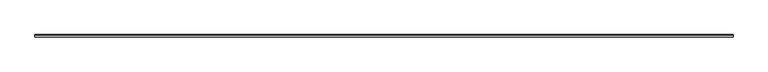
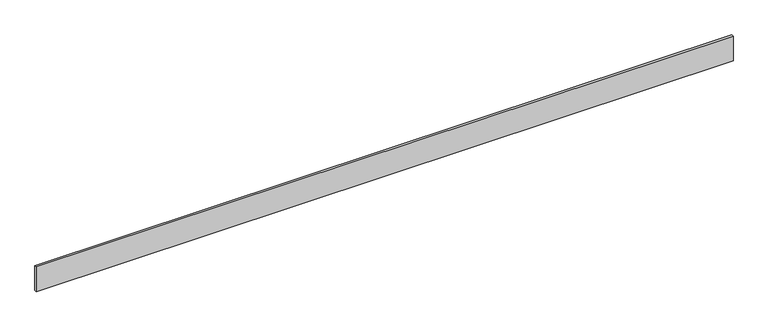
"""IFC4 building model written with IfcOpenShell, lengths in millimetres: proxy geometry, Generic Models 7:Generic Models 1:8:Generic Models 1:8 : Generic Models 7:Generic Models 1:337419:5 : Generic Models 7:Generic Models 1:8:Generic Models 1:8 : Generic Models 7:Generic Models 1:337419:315935."""

from ifc_helpers import new_model, si_unit, frame, origin, place, context, project, spatial, polyline, outline, extrude, source, transform, mapped, element, save


def generic_models_05c8018c(model_context):
    return source(origin(), model_context, "Body", "SweptSolid", [
        extrude(outline(polyline([(-579080.8776331, 3903.4402499), (-579080.0663873, 3902.6290041), (-579080.0663873, 3720.3062499), (-579095.9413873, 3720.3062499), (-579095.9413873, 3903.4402499), (-579080.8776331, 3903.4402499)])), frame((591306.0367239, 0.0, 0.0), z_axis=(1.0, 0.0, 0.0), x_axis=(0.0, 1.0, 0.0)), (0.0, 0.0, 1.0), 4876.8),
    ])


if __name__ == "__main__":
    model = new_model("IFC4")
    model_context = context("Model", 3, world=origin())
    ifc_project = project(units=[si_unit("LENGTHUNIT", "METRE", prefix="MILLI")], contexts=[model_context])
    site = spatial("IfcSite", under=ifc_project)
    building = spatial("IfcBuilding", under=site)
    placement = place(None, origin())
    generic_models_shape = generic_models_05c8018c(model_context)
    element("IfcBuildingElementProxy", 1, Name="Generic Models 7:Generic Models 1:8:Generic Models 1:8 : Generic Models 7:Generic Models 1:337419:5 : Generic Models 7:Generic Models 1:8:Generic Models 1:8 : Generic Models 7:Generic Models 1:337419:315935", ObjectType="Generic Models 7:Generic Models 1:8:Generic Models 1:8 : Generic Models 7:Generic Models 1:337419:5 : Generic Models 7:Generic Models 1:8:Generic Models 1:8 : Generic Models 7:Generic Models 1:337419:315935", at=placement, inside=building, context=model_context, shape_type="MappedRepresentation", body=[
        mapped(generic_models_shape, transform((0.0, 0.0, 0.0), x_axis=(1.0, 0.0, 0.0), y_axis=(0.0, 1.0, 0.0), z_axis=(0.0, 0.0, 1.0))),
    ])
    save(model, "model.ifc")

# Revit data of these elements
# Type "Generic Models 7:Generic Models 1:8:Generic Models 1:8 : Generic Models 7:Generic Models 1:337419:5 : Generic Models 7:Generic Models 1:8:Generic Models 1:8 : Generic Models 7:Generic Models 1:337419:315935"
#   NameOverride = "Generic Models 7:Generic Models 1:8:Generic Models 1:8 : Generic Models 7:Generic Models 1:337419:315935"
#   ObjectTypeOverride = "Generic Models 1:8 : Generic Models 7:Generic Models 1:337419"
#   Reference = "Generic Models 1"
#   Tag = "315935"
# Element 1 (IfcBuildingElementProxy, "Generic Models 7:Generic Models 1:8:Generic Models 1:8 : Generic Models 7:Generic Models 1:337419:5 : Generic Models 7:Generic Models 1:8:Generic Models 1:8 : Generic Models 7:Generic Models 1:337419:315935")
#   Materials on its faces: "ENGINEERED WOOD TRIM (LP SMARTSIDE)"
# Materials
#   "ENGINEERED WOOD TRIM (LP SMARTSIDE)": class "Wood", colour RGB 108 80 40, transparency 0, Description = "Pinus Echinata", Cost = 0
